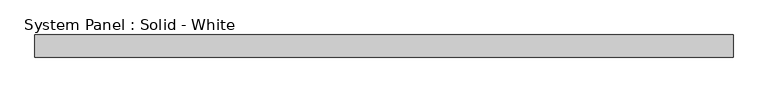
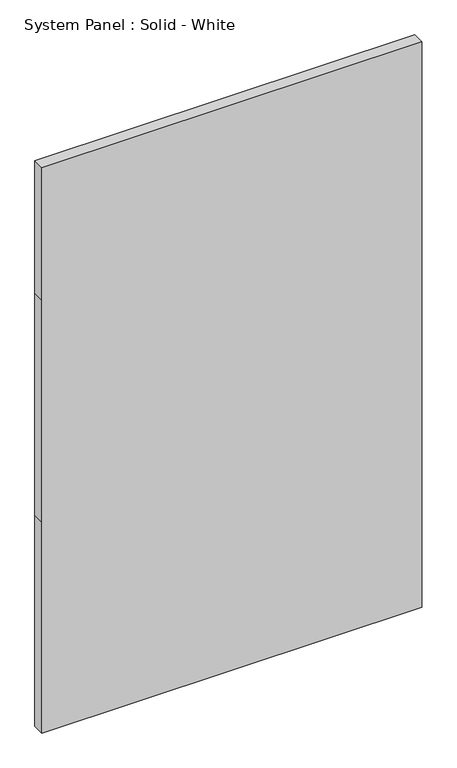
"""IFC4 building model written with IfcOpenShell, lengths in millimetres: plate geometry, System Panel : Solid - White."""

import ifcopenshell
import ifcopenshell.guid

model = None  # the IFC model being written
_history = None  # IfcOwnerHistory: only IFC2X3 demands one
_inside = {}  # id of a spatial element -> (the spatial element, [elements in it])
_under = {}  # id of a project, library or spatial element -> (it, [spatial elements below it])
_declared = {}  # id of a project -> (the project, [libraries it declares])
_typed = {}  # id of a type object -> (the type object, [elements of that type])
_made_of = {}  # id of a material, layer set ... -> (it, [elements and type objects made of it])


def new_model(schema):
    """Start an empty IFC model of exactly this schema.

    Asked for "IFC4X3", IfcOpenShell would pick the latest addendum, in which some entities
    have other attributes; the version numbers below select the first issue.
    IFC2X3 requires an IfcOwnerHistory on every rooted entity: one is made here for all.
    """
    global model, _history
    if schema == "IFC4X3":
        model = ifcopenshell.file(schema_version=(4, 3, 0, 0))
    else:
        model = ifcopenshell.file(schema=schema)
    _inside.clear()
    _under.clear()
    _declared.clear()
    _typed.clear()
    _made_of.clear()
    _history = None
    if model.schema == "IFC2X3":
        org = make("IfcOrganization", Name="unknown")
        user = make(
            "IfcPersonAndOrganization",
            ThePerson=make("IfcPerson", FamilyName="unknown"),
            TheOrganization=org,
        )
        app = make(
            "IfcApplication",
            ApplicationDeveloper=org,
            Version="unknown",
            ApplicationFullName="unknown",
            ApplicationIdentifier="unknown",
        )
        _history = make(
            "IfcOwnerHistory",
            OwningUser=user,
            OwningApplication=app,
            ChangeAction="ADDED",
            CreationDate=0,
        )
    return model


def make(cls, **values):
    """One entity of the class cls with the attributes given. An attribute that is None is left unset."""
    return model.create_entity(
        cls, **{name: value for name, value in values.items() if value is not None}
    )


def rooted(cls, **values):
    """An entity with a GlobalId (a new one), such as an element, a storey or a relation."""
    return make(cls, GlobalId=ifcopenshell.guid.new(), OwnerHistory=_history, **values)


def si_unit(unit_type, name, prefix=None):
    """IfcSIUnit, for example si_unit("LENGTHUNIT", "METRE", prefix="MILLI")."""
    return make("IfcSIUnit", UnitType=unit_type, Prefix=prefix, Name=name)


def assignment(units):
    """IfcUnitAssignment: the units of a project."""
    return None if units is None else make("IfcUnitAssignment", Units=units)


def point(xyz):
    """IfcCartesianPoint."""
    return None if xyz is None else make("IfcCartesianPoint", Coordinates=xyz)


def direction(xyz):
    """IfcDirection."""
    return None if xyz is None else make("IfcDirection", DirectionRatios=xyz)


def frame(location, z_axis=None, x_axis=None):
    """IfcAxis2Placement3D, a coordinate frame: its origin and axes. An axis left out is left unset."""
    return make(
        "IfcAxis2Placement3D",
        Location=point(location),
        Axis=direction(z_axis),
        RefDirection=direction(x_axis),
    )


def origin():
    """The frame at (0, 0, 0) with its axes left unset."""
    return frame((0.0, 0.0, 0.0))


def place(relative_to, where):
    """IfcLocalPlacement: puts the frame where relative to a parent placement (None: the world)."""
    return make(
        "IfcLocalPlacement", PlacementRelTo=relative_to, RelativePlacement=where
    )


def context(
    kind, dimensions, precision=None, world=None, true_north=None, identifier=None
):
    """IfcGeometricRepresentationContext, for example the 3D "Model" context."""
    return make(
        "IfcGeometricRepresentationContext",
        ContextIdentifier=identifier,
        ContextType=kind,
        CoordinateSpaceDimension=dimensions,
        Precision=precision,
        WorldCoordinateSystem=world,
        TrueNorth=true_north,
    )


def project(units=None, contexts=None):
    """IfcProject with its units and contexts."""
    return rooted(
        "IfcProject",
        Name="project",
        RepresentationContexts=contexts,
        UnitsInContext=assignment(units),
    )


def spatial(cls, under=None, at=None, **own):
    """A site, building, storey or space (cls), placed at a placement, below another one or the project."""
    s = rooted(cls, ObjectPlacement=at, **own)
    if under is not None:
        _under.setdefault(under.id(), (under, []))[1].append(s)
    return s


def polyline(points):
    """IfcPolyline through the points."""
    return make("IfcPolyline", Points=[point(p) for p in points])


def outline(outer, holes=None, kind="AREA"):
    """IfcArbitraryClosedProfileDef: a profile drawn as a closed curve; with holes, ...WithVoids."""
    if holes is None:
        return make("IfcArbitraryClosedProfileDef", ProfileType=kind, OuterCurve=outer)
    return make(
        "IfcArbitraryProfileDefWithVoids",
        ProfileType=kind,
        OuterCurve=outer,
        InnerCurves=holes,
    )


def extrude(swept, where, along, depth):
    """IfcExtrudedAreaSolid: the profile swept, set in the frame where, extruded along a direction by depth."""
    return make(
        "IfcExtrudedAreaSolid",
        SweptArea=swept,
        Position=where,
        ExtrudedDirection=direction(along),
        Depth=depth,
    )


def shape(context_of_items, identifier, shape_type, items):
    """IfcShapeRepresentation: the items that make up one representation, for example the "Body"."""
    return make(
        "IfcShapeRepresentation",
        ContextOfItems=context_of_items,
        RepresentationIdentifier=identifier,
        RepresentationType=shape_type,
        Items=items,
    )


def source(mapping_origin, context_of_items, identifier, shape_type, items):
    """IfcRepresentationMap: a shape defined once, which mapped items show again and again."""
    return make(
        "IfcRepresentationMap",
        MappingOrigin=mapping_origin,
        MappedRepresentation=shape(context_of_items, identifier, shape_type, items),
    )


def transform(
    local_origin,
    x_axis=None,
    y_axis=None,
    z_axis=None,
    scale=None,
    scale2=None,
    scale3=None,
    uniform=True,
):
    """IfcCartesianTransformationOperator3D, or its non-uniform kind. x_axis, y_axis, z_axis: its Axis1, 2, 3."""
    if uniform:
        return make(
            "IfcCartesianTransformationOperator3D",
            Axis1=direction(x_axis),
            Axis2=direction(y_axis),
            LocalOrigin=point(local_origin),
            Scale=scale,
            Axis3=direction(z_axis),
        )
    return make(
        "IfcCartesianTransformationOperator3DnonUniform",
        Axis1=direction(x_axis),
        Axis2=direction(y_axis),
        LocalOrigin=point(local_origin),
        Scale=scale,
        Axis3=direction(z_axis),
        Scale2=scale2,
        Scale3=scale3,
    )


def mapped(mapping_source, mapping_target):
    """IfcMappedItem: shows the shape of a source again, moved by a transform."""
    return make(
        "IfcMappedItem", MappingSource=mapping_source, MappingTarget=mapping_target
    )


def made_of(thing, what):
    """Note that an element or type object is made of a material, layer set ...; save() writes the relation."""
    if what is not None:
        _made_of.setdefault(what.id(), (what, []))[1].append(thing)
    return thing


def element(
    cls,
    number,
    at=None,
    inside=None,
    cuts=None,
    type_object=None,
    material=None,
    context=None,
    identifier="Body",
    shape_type=None,
    held_by="IfcProductDefinitionShape",
    body=None,
    shapes=None,
    **own,
):
    """One element of the class cls, such as IfcWall. Its Tag is "e" and its number.

    at: its placement. inside: the storey or other place that contains it. cuts: it is an
    opening in that element (IfcRelVoidsElement). A single representation is given by context,
    identifier, shape_type and body (its items); several are given by shapes. held_by: the class
    of the entity that holds the representations. save() writes the other relations.
    """
    e = rooted(cls, Tag="e%d" % number, ObjectPlacement=at, **own)
    if body is not None:
        shapes = [shape(context, identifier, shape_type, body)]
    if shapes is not None:
        e.Representation = make(held_by, Representations=shapes)
    if inside is not None:
        _inside.setdefault(inside.id(), (inside, []))[1].append(e)
    if cuts is not None:
        rooted(
            "IfcRelVoidsElement", RelatingBuildingElement=cuts, RelatedOpeningElement=e
        )
    if type_object is not None:
        _typed.setdefault(type_object.id(), (type_object, []))[1].append(e)
    return made_of(e, material)


def aggregate(whole, parts):
    """IfcRelAggregates: a whole, such as a stair, and the parts it consists of."""
    return rooted("IfcRelAggregates", RelatingObject=whole, RelatedObjects=parts)


def save(model, path):
    """Write the relations noted so far, then the file.

    IfcRelAggregates (storeys below a building ...), IfcRelContainedInSpatialStructure (elements
    in a storey), IfcRelDefinesByType, IfcRelAssociatesMaterial and IfcRelDeclares: one each for
    every whole, place, type object, material and project.
    """
    for whole, parts in _under.values():
        aggregate(whole, parts)
    for where, things in _inside.values():
        rooted(
            "IfcRelContainedInSpatialStructure",
            RelatedElements=things,
            RelatingStructure=where,
        )
    for kind, things in _typed.values():
        rooted("IfcRelDefinesByType", RelatedObjects=things, RelatingType=kind)
    for what, things in _made_of.values():
        rooted("IfcRelAssociatesMaterial", RelatedObjects=things, RelatingMaterial=what)
    for by, libraries in _declared.values():
        rooted("IfcRelDeclares", RelatingContext=by, RelatedDefinitions=libraries)
    model.write(path)


def system_panel_solid_white_b427edf1(model_context):
    return source(origin(), model_context, "Body", "SweptSolid", [
        extrude(outline(polyline([(0.0, -985.4757062), (0.0, 985.4757062), (1155.7, 985.4757062), (2374.9, 985.4757062), (3101.9419949, 985.4757062), (3101.9419949, -985.4757062), (2374.9, -985.4757062), (1155.7, -985.4757062), (0.0, -985.4757062)])), frame((0.0, -44.45, 0.0), z_axis=(0.0, 1.0, 0.0), x_axis=(0.0, 0.0, 1.0)), (0.0, 0.0, 1.0), 63.5),
    ])


if __name__ == "__main__":
    model = new_model("IFC4")
    model_context = context("Model", 3, world=origin())
    ifc_project = project(units=[si_unit("LENGTHUNIT", "METRE", prefix="MILLI")], contexts=[model_context])
    site = spatial("IfcSite", under=ifc_project)
    building = spatial("IfcBuilding", under=site)
    placement = place(None, origin())
    system_panel_solid_white_shape = system_panel_solid_white_b427edf1(model_context)
    element("IfcPlate", 1, ObjectType="System Panel : Solid - White", at=placement, inside=building, context=model_context, shape_type="MappedRepresentation", body=[
        mapped(system_panel_solid_white_shape, transform((0.0, 0.0, 0.0), x_axis=(1.0, 0.0, 0.0), y_axis=(0.0, 1.0, 0.0), z_axis=(0.0, 0.0, 1.0))),
    ])
    save(model, "model.ifc")

# Revit data of these elements
# Element 1 (IfcPlate, "System Panel : Solid - White")
#   Materials on its faces: "White Panel"
# Materials
#   "White Panel": class "Unassigned", colour RGB 255 255 255, transparency 0
